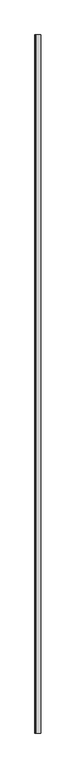
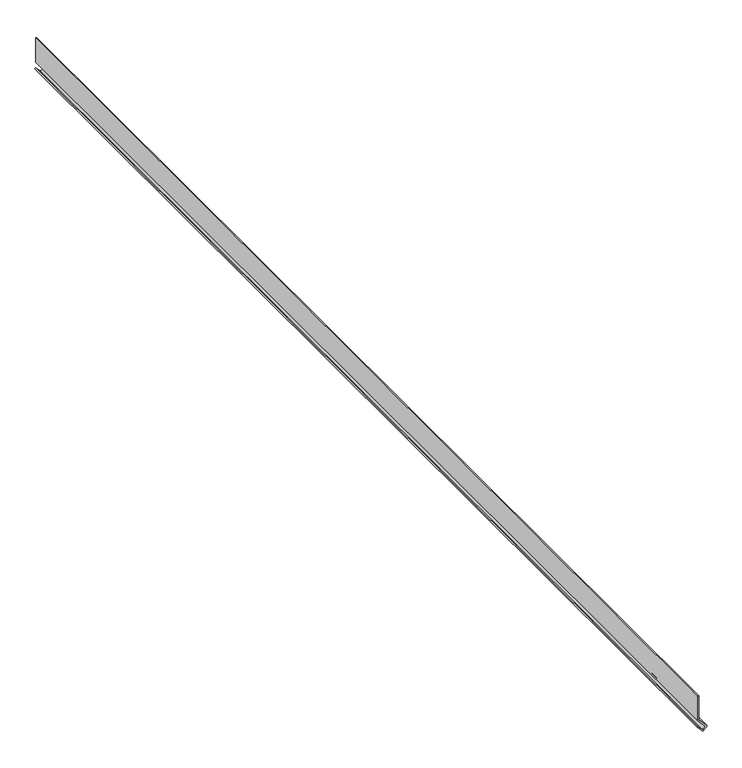
"""IFC4 building model written with IfcOpenShell, lengths in millimetres: proxy geometry, Flashing021 11290 : Flashing021 11290."""

from ifc_helpers import new_model, si_unit, frame, origin, place, context, project, spatial, polyline, outline, extrude, source, transform, mapped, element, save


def generic_models_f64f48d8(model_context):
    return source(origin(), model_context, "Body", "SweptSolid", [
        extrude(outline(polyline([(43008.8710938, 16651.7480469), (42993.6445313, 16665.2148438), (42989.0546875, 16660.4316406), (42998.2304688, 16652.1347656), (42996.8890886, 16650.6512902), (42986.1852076, 16660.3298953), (42993.5310498, 16667.9852007), (43009.6286352, 16653.7480469), (43053.53125, 16653.7480469), (43053.53125, 16651.7480469), (43008.8710938, 16651.7480469)])), frame((0.0, 7982.1435673, 0.0), z_axis=(0.0, 1.0, 0.0), x_axis=(0.0, 0.0, 1.0)), (0.0, 0.0, 1.0), 2000.0),
    ])


if __name__ == "__main__":
    model = new_model("IFC4")
    model_context = context("Model", 3, world=origin())
    ifc_project = project(units=[si_unit("LENGTHUNIT", "METRE", prefix="MILLI")], contexts=[model_context])
    site = spatial("IfcSite", under=ifc_project)
    building = spatial("IfcBuilding", under=site)
    placement = place(None, origin())
    generic_models_shape = generic_models_f64f48d8(model_context)
    element("IfcBuildingElementProxy", 1, Name="Flashing021 11290 : Flashing021 11290", ObjectType="Flashing021 11290 : Flashing021 11290", at=placement, inside=building, context=model_context, shape_type="MappedRepresentation", body=[
        mapped(generic_models_shape, transform((0.0, 0.0, 0.0), x_axis=(1.0, 0.0, 0.0), y_axis=(0.0, 1.0, 0.0), z_axis=(0.0, 0.0, 1.0))),
    ])
    save(model, "model.ifc")

# Revit data of these elements
# Type "Flashing021 11290 : Flashing021 11290"
#   NameOverride = "Flashing021"
# Element 1 (IfcBuildingElementProxy, "Flashing021 11290 : Flashing021 11290")
#   Materials on its faces: "16GA. COPPER BRAKE METAL FLASHING"
# Materials
#   "16GA. COPPER BRAKE METAL FLASHING": class "Unassigned", colour RGB 128 128 128, transparency 0
